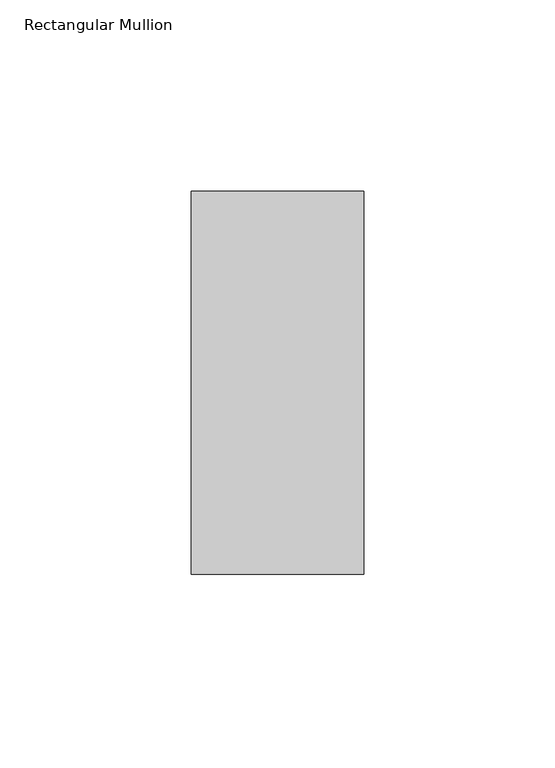
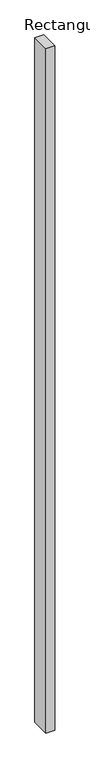
"""IFC4 building model written with IfcOpenShell, lengths in millimetres: member geometry, Rectangular Mullion : 알루미늄_Rectangular Cap_100 x 45."""

import ifcopenshell
import ifcopenshell.guid

model = None  # the IFC model being written
_history = None  # IfcOwnerHistory: only IFC2X3 demands one
_inside = {}  # id of a spatial element -> (the spatial element, [elements in it])
_under = {}  # id of a project, library or spatial element -> (it, [spatial elements below it])
_declared = {}  # id of a project -> (the project, [libraries it declares])
_typed = {}  # id of a type object -> (the type object, [elements of that type])
_made_of = {}  # id of a material, layer set ... -> (it, [elements and type objects made of it])


def new_model(schema):
    """Start an empty IFC model of exactly this schema.

    Asked for "IFC4X3", IfcOpenShell would pick the latest addendum, in which some entities
    have other attributes; the version numbers below select the first issue.
    IFC2X3 requires an IfcOwnerHistory on every rooted entity: one is made here for all.
    """
    global model, _history
    if schema == "IFC4X3":
        model = ifcopenshell.file(schema_version=(4, 3, 0, 0))
    else:
        model = ifcopenshell.file(schema=schema)
    _inside.clear()
    _under.clear()
    _declared.clear()
    _typed.clear()
    _made_of.clear()
    _history = None
    if model.schema == "IFC2X3":
        org = make("IfcOrganization", Name="unknown")
        user = make(
            "IfcPersonAndOrganization",
            ThePerson=make("IfcPerson", FamilyName="unknown"),
            TheOrganization=org,
        )
        app = make(
            "IfcApplication",
            ApplicationDeveloper=org,
            Version="unknown",
            ApplicationFullName="unknown",
            ApplicationIdentifier="unknown",
        )
        _history = make(
            "IfcOwnerHistory",
            OwningUser=user,
            OwningApplication=app,
            ChangeAction="ADDED",
            CreationDate=0,
        )
    return model


def make(cls, **values):
    """One entity of the class cls with the attributes given. An attribute that is None is left unset."""
    return model.create_entity(
        cls, **{name: value for name, value in values.items() if value is not None}
    )


def rooted(cls, **values):
    """An entity with a GlobalId (a new one), such as an element, a storey or a relation."""
    return make(cls, GlobalId=ifcopenshell.guid.new(), OwnerHistory=_history, **values)


def si_unit(unit_type, name, prefix=None):
    """IfcSIUnit, for example si_unit("LENGTHUNIT", "METRE", prefix="MILLI")."""
    return make("IfcSIUnit", UnitType=unit_type, Prefix=prefix, Name=name)


def assignment(units):
    """IfcUnitAssignment: the units of a project."""
    return None if units is None else make("IfcUnitAssignment", Units=units)


def point(xyz):
    """IfcCartesianPoint."""
    return None if xyz is None else make("IfcCartesianPoint", Coordinates=xyz)


def direction(xyz):
    """IfcDirection."""
    return None if xyz is None else make("IfcDirection", DirectionRatios=xyz)


def frame(location, z_axis=None, x_axis=None):
    """IfcAxis2Placement3D, a coordinate frame: its origin and axes. An axis left out is left unset."""
    return make(
        "IfcAxis2Placement3D",
        Location=point(location),
        Axis=direction(z_axis),
        RefDirection=direction(x_axis),
    )


def origin():
    """The frame at (0, 0, 0) with its axes left unset."""
    return frame((0.0, 0.0, 0.0))


def place(relative_to, where):
    """IfcLocalPlacement: puts the frame where relative to a parent placement (None: the world)."""
    return make(
        "IfcLocalPlacement", PlacementRelTo=relative_to, RelativePlacement=where
    )


def context(
    kind, dimensions, precision=None, world=None, true_north=None, identifier=None
):
    """IfcGeometricRepresentationContext, for example the 3D "Model" context."""
    return make(
        "IfcGeometricRepresentationContext",
        ContextIdentifier=identifier,
        ContextType=kind,
        CoordinateSpaceDimension=dimensions,
        Precision=precision,
        WorldCoordinateSystem=world,
        TrueNorth=true_north,
    )


def project(units=None, contexts=None):
    """IfcProject with its units and contexts."""
    return rooted(
        "IfcProject",
        Name="project",
        RepresentationContexts=contexts,
        UnitsInContext=assignment(units),
    )


def spatial(cls, under=None, at=None, **own):
    """A site, building, storey or space (cls), placed at a placement, below another one or the project."""
    s = rooted(cls, ObjectPlacement=at, **own)
    if under is not None:
        _under.setdefault(under.id(), (under, []))[1].append(s)
    return s


def polyline(points):
    """IfcPolyline through the points."""
    return make("IfcPolyline", Points=[point(p) for p in points])


def outline(outer, holes=None, kind="AREA"):
    """IfcArbitraryClosedProfileDef: a profile drawn as a closed curve; with holes, ...WithVoids."""
    if holes is None:
        return make("IfcArbitraryClosedProfileDef", ProfileType=kind, OuterCurve=outer)
    return make(
        "IfcArbitraryProfileDefWithVoids",
        ProfileType=kind,
        OuterCurve=outer,
        InnerCurves=holes,
    )


def extrude(swept, where, along, depth):
    """IfcExtrudedAreaSolid: the profile swept, set in the frame where, extruded along a direction by depth."""
    return make(
        "IfcExtrudedAreaSolid",
        SweptArea=swept,
        Position=where,
        ExtrudedDirection=direction(along),
        Depth=depth,
    )


def shape(context_of_items, identifier, shape_type, items):
    """IfcShapeRepresentation: the items that make up one representation, for example the "Body"."""
    return make(
        "IfcShapeRepresentation",
        ContextOfItems=context_of_items,
        RepresentationIdentifier=identifier,
        RepresentationType=shape_type,
        Items=items,
    )


def source(mapping_origin, context_of_items, identifier, shape_type, items):
    """IfcRepresentationMap: a shape defined once, which mapped items show again and again."""
    return make(
        "IfcRepresentationMap",
        MappingOrigin=mapping_origin,
        MappedRepresentation=shape(context_of_items, identifier, shape_type, items),
    )


def transform(
    local_origin,
    x_axis=None,
    y_axis=None,
    z_axis=None,
    scale=None,
    scale2=None,
    scale3=None,
    uniform=True,
):
    """IfcCartesianTransformationOperator3D, or its non-uniform kind. x_axis, y_axis, z_axis: its Axis1, 2, 3."""
    if uniform:
        return make(
            "IfcCartesianTransformationOperator3D",
            Axis1=direction(x_axis),
            Axis2=direction(y_axis),
            LocalOrigin=point(local_origin),
            Scale=scale,
            Axis3=direction(z_axis),
        )
    return make(
        "IfcCartesianTransformationOperator3DnonUniform",
        Axis1=direction(x_axis),
        Axis2=direction(y_axis),
        LocalOrigin=point(local_origin),
        Scale=scale,
        Axis3=direction(z_axis),
        Scale2=scale2,
        Scale3=scale3,
    )


def mapped(mapping_source, mapping_target):
    """IfcMappedItem: shows the shape of a source again, moved by a transform."""
    return make(
        "IfcMappedItem", MappingSource=mapping_source, MappingTarget=mapping_target
    )


def made_of(thing, what):
    """Note that an element or type object is made of a material, layer set ...; save() writes the relation."""
    if what is not None:
        _made_of.setdefault(what.id(), (what, []))[1].append(thing)
    return thing


def element(
    cls,
    number,
    at=None,
    inside=None,
    cuts=None,
    type_object=None,
    material=None,
    context=None,
    identifier="Body",
    shape_type=None,
    held_by="IfcProductDefinitionShape",
    body=None,
    shapes=None,
    **own,
):
    """One element of the class cls, such as IfcWall. Its Tag is "e" and its number.

    at: its placement. inside: the storey or other place that contains it. cuts: it is an
    opening in that element (IfcRelVoidsElement). A single representation is given by context,
    identifier, shape_type and body (its items); several are given by shapes. held_by: the class
    of the entity that holds the representations. save() writes the other relations.
    """
    e = rooted(cls, Tag="e%d" % number, ObjectPlacement=at, **own)
    if body is not None:
        shapes = [shape(context, identifier, shape_type, body)]
    if shapes is not None:
        e.Representation = make(held_by, Representations=shapes)
    if inside is not None:
        _inside.setdefault(inside.id(), (inside, []))[1].append(e)
    if cuts is not None:
        rooted(
            "IfcRelVoidsElement", RelatingBuildingElement=cuts, RelatedOpeningElement=e
        )
    if type_object is not None:
        _typed.setdefault(type_object.id(), (type_object, []))[1].append(e)
    return made_of(e, material)


def aggregate(whole, parts):
    """IfcRelAggregates: a whole, such as a stair, and the parts it consists of."""
    return rooted("IfcRelAggregates", RelatingObject=whole, RelatedObjects=parts)


def save(model, path):
    """Write the relations noted so far, then the file.

    IfcRelAggregates (storeys below a building ...), IfcRelContainedInSpatialStructure (elements
    in a storey), IfcRelDefinesByType, IfcRelAssociatesMaterial and IfcRelDeclares: one each for
    every whole, place, type object, material and project.
    """
    for whole, parts in _under.values():
        aggregate(whole, parts)
    for where, things in _inside.values():
        rooted(
            "IfcRelContainedInSpatialStructure",
            RelatedElements=things,
            RelatingStructure=where,
        )
    for kind, things in _typed.values():
        rooted("IfcRelDefinesByType", RelatedObjects=things, RelatingType=kind)
    for what, things in _made_of.values():
        rooted("IfcRelAssociatesMaterial", RelatedObjects=things, RelatingMaterial=what)
    for by, libraries in _declared.values():
        rooted("IfcRelDeclares", RelatingContext=by, RelatedDefinitions=libraries)
    model.write(path)


def rectangular_mullion_03c4161e(model_context):
    return source(origin(), model_context, "Body", "SweptSolid", [
        extrude(outline(polyline([(0.0, 50.0), (0.0, -50.0), (-45.0, -50.0), (-45.0, 50.0), (0.0, 50.0)])), frame((0.0, 0.0, -3775.0), z_axis=(0.0, 0.0, 1.0), x_axis=(1.0, 0.0, 0.0)), (0.0, 0.0, 1.0), 3775.0),
    ])


if __name__ == "__main__":
    model = new_model("IFC4")
    model_context = context("Model", 3, world=origin())
    ifc_project = project(units=[si_unit("LENGTHUNIT", "METRE", prefix="MILLI")], contexts=[model_context])
    site = spatial("IfcSite", under=ifc_project)
    building = spatial("IfcBuilding", under=site)
    placement = place(None, origin())
    rectangular_mullion_shape = rectangular_mullion_03c4161e(model_context)
    element("IfcMember", 1, ObjectType="Rectangular Mullion : 알루미늄_Rectangular Cap_100 x 45", at=placement, inside=building, context=model_context, shape_type="MappedRepresentation", body=[
        mapped(rectangular_mullion_shape, transform((0.0, 0.0, 0.0), x_axis=(1.0, 0.0, 0.0), y_axis=(0.0, 1.0, 0.0), z_axis=(0.0, 0.0, 1.0))),
    ])
    save(model, "model.ifc")

# Revit data of these elements
# Type "Rectangular Mullion : 알루미늄_Rectangular Cap_100 x 45"
#   built-in parameter 1007304 = 0.328084 (stored number, unit not read)
#   built-in parameter 1007301 = 0.0738189 (stored number, unit not read)
#   built-in parameter 1007300 = 0.0738189 (stored number, unit not read)
# Element 1 (IfcMember, "Rectangular Mullion : 알루미늄_Rectangular Cap_100 x 45")
#   Materials on its faces: "00_Metal_Stainless Steel"
# Materials
#   "00_Metal_Stainless Steel": class "Metal", colour RGB 148 148 148, transparency 0, Description = "Steel", Cost = 0
